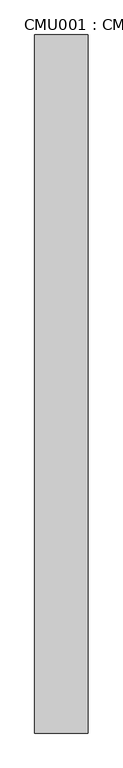
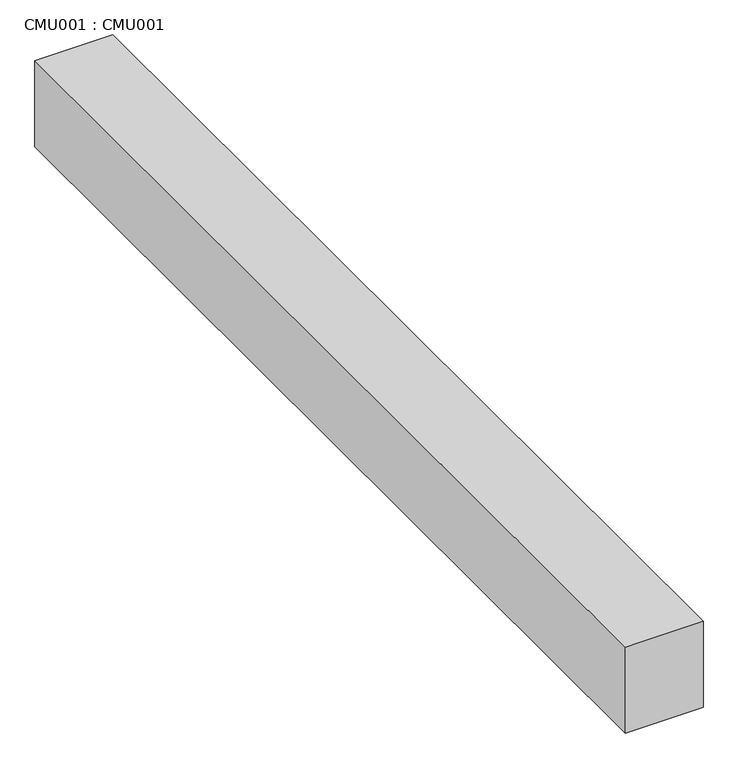
"""IFC4 building model written with IfcOpenShell, lengths in millimetres: proxy geometry, CMU001 : CMU001."""

from ifc_helpers import new_model, si_unit, frame, origin, place, context, project, spatial, polyline, outline, extrude, source, transform, mapped, element, save


def cmu001_cmu001_1df0cabd(model_context):
    return source(origin(), model_context, "Body", "SweptSolid", [
        extrude(outline(polyline([(-10098.4737014, 7982.1531721), (-10250.8737014, 7982.1531721), (-10250.8737014, 9982.1531721), (-10098.4737014, 9982.1531721), (-10098.4737014, 7982.1531721)])), frame((0.0, 0.0, 32819.0563498), z_axis=(0.0, 0.0, 1.0), x_axis=(1.0, 0.0, 0.0)), (0.0, 0.0, 1.0), 177.8),
    ])


if __name__ == "__main__":
    model = new_model("IFC4")
    model_context = context("Model", 3, world=origin())
    ifc_project = project(units=[si_unit("LENGTHUNIT", "METRE", prefix="MILLI")], contexts=[model_context])
    site = spatial("IfcSite", under=ifc_project)
    building = spatial("IfcBuilding", under=site)
    placement = place(None, origin())
    cmu001_cmu001_shape = cmu001_cmu001_1df0cabd(model_context)
    element("IfcBuildingElementProxy", 1, Name="CMU001 : CMU001", ObjectType="CMU001 : CMU001", at=placement, inside=building, context=model_context, shape_type="MappedRepresentation", body=[
        mapped(cmu001_cmu001_shape, transform((0.0, 0.0, 0.0), x_axis=(1.0, 0.0, 0.0), y_axis=(0.0, 1.0, 0.0), z_axis=(0.0, 0.0, 1.0))),
    ])
    save(model, "model.ifc")

# Revit data of these elements
# Type "CMU001 : CMU001"
#   NameOverride = "CMU001"
# Element 1 (IfcBuildingElementProxy, "CMU001 : CMU001")
#   Materials on its faces: "4\" CMU WALL"
# Materials
#   "4\" CMU WALL": class "Unassigned", colour RGB 128 128 128, transparency 0, Cost = 0
